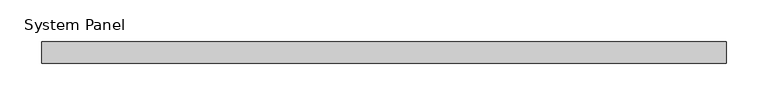
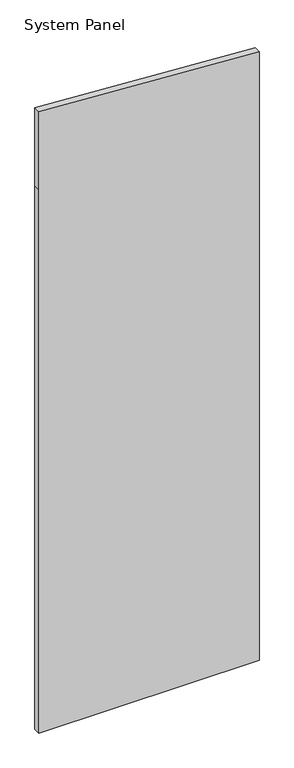
"""IFC4 building model written with IfcOpenShell, lengths in millimetres: plate geometry, System Panel : TEMPERED INSULATED GLAZING (CARDINAL GLASS LoĒ²-240."""

from ifc_helpers import new_model, si_unit, frame, origin, place, context, project, spatial, polyline, outline, extrude, source, transform, mapped, element, save


def system_panel_2ac19692(model_context):
    return source(origin(), model_context, "Body", "SweptSolid", [
        extrude(outline(polyline([(0.0, -407.4278978), (0.0, 407.4278978), (2127.25, 407.4278978), (2380.7247345, 407.4278978), (2431.6532217, -407.4278978), (2127.25, -407.4278978), (0.0, -407.4278978)])), frame((0.0, 6.35, 0.0), z_axis=(0.0, 1.0, 0.0), x_axis=(0.0, 0.0, 1.0)), (0.0, 0.0, 1.0), 25.4),
    ])


if __name__ == "__main__":
    model = new_model("IFC4")
    model_context = context("Model", 3, world=origin())
    ifc_project = project(units=[si_unit("LENGTHUNIT", "METRE", prefix="MILLI")], contexts=[model_context])
    site = spatial("IfcSite", under=ifc_project)
    building = spatial("IfcBuilding", under=site)
    placement = place(None, origin())
    system_panel_shape = system_panel_2ac19692(model_context)
    element("IfcPlate", 1, ObjectType="System Panel : TEMPERED INSULATED GLAZING (CARDINAL GLASS LoĒ²-240", at=placement, inside=building, context=model_context, shape_type="MappedRepresentation", body=[
        mapped(system_panel_shape, transform((0.0, 0.0, 0.0), x_axis=(1.0, 0.0, 0.0), y_axis=(0.0, 1.0, 0.0), z_axis=(0.0, 0.0, 1.0))),
    ])
    save(model, "model.ifc")

# Revit data of these elements
# Type "System Panel : TEMPERED INSULATED GLAZING (CARDINAL GLASS LoĒ²-240"
#   Construction Type Id = "opn-s72"
#   Analytic Construction = "Double glazing - 1/4 in thick - low-E/clear (e = 0.1) glass"
#   Visual Light Transmittance = 0.72
#   Solar Heat Gain Coefficient = 0.6
#   Heat Transfer Coefficient (U) = 1.9873 W/(m²·K)
#   Transparency_Hack = 70
# Element 1 (IfcPlate, "System Panel : TEMPERED INSULATED GLAZING (CARDINAL GLASS LoĒ²-240")
#   Materials on its faces: "TEMPERED INSULATED GLAZING (CARDINAL GLASS LoĒ²-240\nOR EQUIVALENT)"
# Materials
#   "TEMPERED INSULATED GLAZING (CARDINAL GLASS LoĒ²-240\nOR EQUIVALENT)": class "Glass", colour RGB 196 205 210, transparency 0.85, Description = "Soda Lime Glass", Cost = 0
